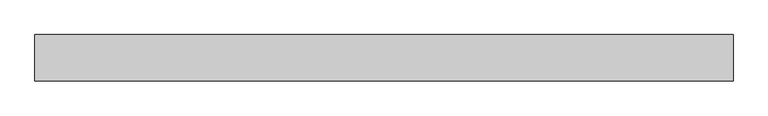
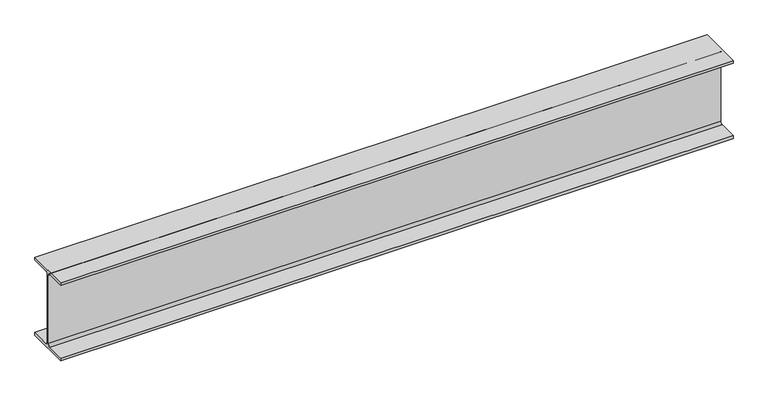
"""IFC4 building model written with IfcOpenShell, lengths in millimetres: beam geometry, Old_Steel Beam_H-KSD3502 : H_SB_ASB_H-250×125x6x9."""

from ifc_helpers import new_model, si_unit, point, frame, frame_2d, origin, place, context, project, spatial, polyline, circle_curve, trimmed, segment, composite_curve, outline, extrude, source, transform, mapped, element, save


def beam_33eac880(model_context):
    return source(origin(), model_context, "Body", "SweptSolid", [
        extrude(outline(composite_curve([segment(polyline([(82.5, -141.5), (82.5, -151.7), (-82.5, -151.7), (-82.5, -141.5), (-11.9, -141.5)]), True, "CONTINUOUS"), segment(trimmed(circle_curve(frame_2d((-11.9, -132.6)), 8.9), [point((-11.9, -141.5))], [point((-3.0, -132.6))], True, "CARTESIAN"), True, "CONTINUOUS"), segment(polyline([(-3.0, -132.6), (-3.0, 132.6)]), True, "CONTINUOUS"), segment(trimmed(circle_curve(frame_2d((-11.9, 132.6)), 8.9), [point((-3.0, 132.6))], [point((-11.9, 141.5))], True, "CARTESIAN"), True, "CONTINUOUS"), segment(polyline([(-11.9, 141.5), (-82.5, 141.5), (-82.5, 151.7), (82.5, 151.7), (82.5, 141.5), (11.9, 141.5)]), True, "CONTINUOUS"), segment(trimmed(circle_curve(frame_2d((11.9, 132.6)), 8.9), [point((11.9, 141.5))], [point((3.0, 132.6))], True, "CARTESIAN"), True, "CONTINUOUS"), segment(polyline([(3.0, 132.6), (3.0, -132.6)]), True, "CONTINUOUS"), segment(trimmed(circle_curve(frame_2d((11.9, -132.6)), 8.9), [point((3.0, -132.6))], [point((11.9, -141.5))], True, "CARTESIAN"), True, "CONTINUOUS"), segment(polyline([(11.9, -141.5), (82.5, -141.5)]), True, "CONTINUOUS")], self_intersect=False)), frame((-1137.3, 0.0, 0.0), z_axis=(1.0, 0.0, 0.0), x_axis=(0.0, 1.0, 0.0)), (0.0, 0.0, 1.0), 2474.6),
    ])


if __name__ == "__main__":
    model = new_model("IFC4")
    model_context = context("Model", 3, world=origin())
    ifc_project = project(units=[si_unit("LENGTHUNIT", "METRE", prefix="MILLI")], contexts=[model_context])
    site = spatial("IfcSite", under=ifc_project)
    building = spatial("IfcBuilding", under=site)
    placement = place(None, origin())
    beam_shape = beam_33eac880(model_context)
    element("IfcBeam", 1, ObjectType="Old_Steel Beam_H-KSD3502 : H_SB_ASB_H-250×125x6x9", at=placement, inside=building, context=model_context, shape_type="MappedRepresentation", body=[
        mapped(beam_shape, transform((0.0, 0.0, 0.0), x_axis=(1.0, 0.0, 0.0), y_axis=(0.0, 1.0, 0.0), z_axis=(0.0, 0.0, 1.0))),
    ])
    save(model, "model.ifc")

# Revit data of these elements
# Type "Old_Steel Beam_H-KSD3502 : H_SB_ASB_H-250×125x6x9"
#   Width = 12.5 cm
#   Web Thickness = 0.6 cm
#   Web Fillet = 1.2 cm
#   Warping Constant = 42539.8 cm⁶
#   Torsional Moment of Inertia = 7.8102 cm⁴
#   Torsional Modulus = 1.0 cm³
#   Section Area = 37.66 cm²
#   Plastic Modulus weak axis = 73.1 cm³
#   Plastic Modulus strong axis = 366.0 cm³
#   Perimeter = 0.97 m²/m
#   Nominal Weight = 29.60 kgf/m
#   Moment of Inertia weak axis = 294.00 cm⁴
#   Moment of Inertia strong axis = 4050.00 cm⁴
#   Height = 25.0 cm
#   Flange Thickness = 0.9 cm
#   Elastic Modulus weak axis = 47.0 cm³
#   Elastic Modulus strong axis = 324.0 cm³
#   Centroid Vertical = 12.5 cm
#   Centroid Horizontal = 6.25 cm
#   Length [instance default] = 1.5240 m
#   Structural Material [instance default] = Steel, 45-345
#   Assembly Code = ""
# Element 1 (IfcBeam, "Old_Steel Beam_H-KSD3502 : H_SB_ASB_H-250×125x6x9")
#   Structural Material = none
# Materials
#   "Steel, 45-345": class "Metal", colour RGB 189 187 185, transparency 0, Description = "Steel 345 MPa", Cost = 0
